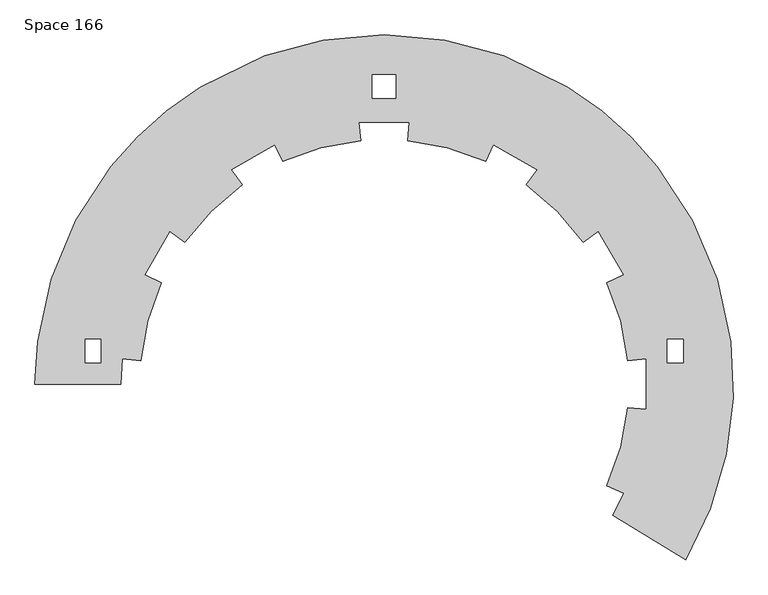
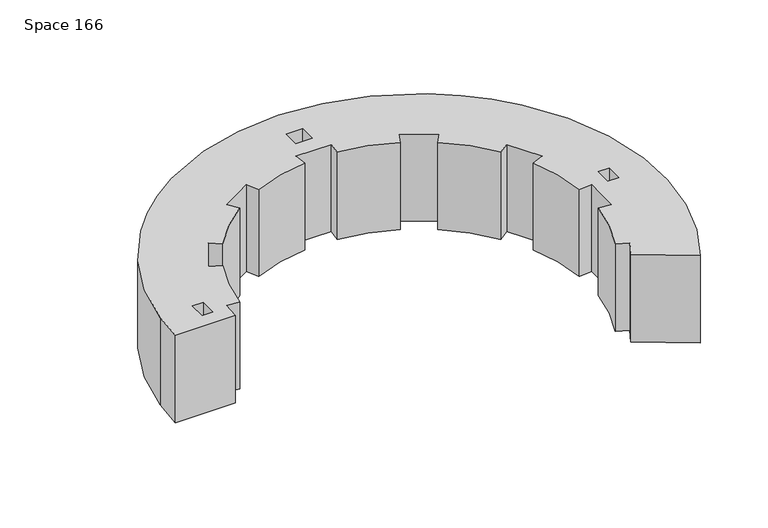
"""IFC4 building model written with IfcOpenShell, lengths in millimetres: proxy geometry, Space 166."""

from ifc_helpers import new_model, si_unit, point, frame_2d, origin, origin_with_axes, place, context, project, spatial, polyline, circle_curve, trimmed, segment, composite_curve, outline, extrude, source, transform, mapped, element, save


def space_166_33292cd7(model_context):
    return source(origin(), model_context, "Body", "SweptSolid", [
        extrude(outline(composite_curve([segment(trimmed(circle_curve(frame_2d((-24639.5440345, -26167.559635)), 5638.8), [point((-19508.4544203, -28505.9318917))], [point((-19026.7039512, -26708.0146643))], True, "CARTESIAN"), True, "CONTINUOUS"), segment(polyline([(-19026.7039512, -26708.0146643), (-18603.2126386, -26748.7922397)]), True, "CONTINUOUS"), segment(trimmed(circle_curve(frame_2d((-24639.5440345, -26167.559635)), 6064.25), [point((-18603.2126386, -26748.7922397))], [point((-18603.2126386, -25586.3270303))], True, "CARTESIAN"), True, "CONTINUOUS"), segment(polyline([(-18603.2126386, -25586.3270303), (-19026.7039512, -25627.1046057)]), True, "CONTINUOUS"), segment(trimmed(circle_curve(frame_2d((-24639.5440345, -26167.559635)), 5638.8), [point((-19026.7039512, -25627.1046057))], [point((-19508.4544203, -23829.1873783))], True, "CARTESIAN"), True, "CONTINUOUS"), segment(polyline([(-19508.4544203, -23829.1873783), (-19121.3113976, -23652.7561382)]), True, "CONTINUOUS"), segment(trimmed(circle_curve(frame_2d((-24639.5440345, -26167.559635)), 6064.25), [point((-19121.3113976, -23652.7561382))], [point((-19702.5440023, -22646.0317359))], True, "CARTESIAN"), True, "CONTINUOUS"), segment(polyline([(-19702.5440023, -22646.0317359), (-20048.9094496, -22893.0918084)]), True, "CONTINUOUS"), segment(trimmed(circle_curve(frame_2d((-24639.5440345, -26167.559635)), 5638.8), [point((-20048.9094496, -22893.0918084))], [point((-21365.0762078, -21576.9250501))], True, "CARTESIAN"), True, "CONTINUOUS"), segment(polyline([(-21365.0762078, -21576.9250501), (-21118.0161353, -21230.5596028)]), True, "CONTINUOUS"), segment(trimmed(circle_curve(frame_2d((-24639.5440345, -26167.559635)), 6064.25), [point((-21118.0161353, -21230.5596028))], [point((-22124.7405377, -20649.3269981))], True, "CARTESIAN"), True, "CONTINUOUS"), segment(polyline([(-22124.7405377, -20649.3269981), (-22301.1717778, -21036.4700208)]), True, "CONTINUOUS"), segment(trimmed(circle_curve(frame_2d((-24639.5440345, -26167.559635)), 5638.8), [point((-22301.1717778, -21036.4700208))], [point((-24099.0890052, -20554.7195517))], True, "CARTESIAN"), True, "CONTINUOUS"), segment(polyline([(-24099.0890052, -20554.7195517), (-24058.3114298, -20131.2282391)]), True, "CONTINUOUS"), segment(trimmed(circle_curve(frame_2d((-24639.5440345, -26167.559635)), 6064.25), [point((-24058.3114298, -20131.2282391))], [point((-25220.7766392, -20131.2282391))], True, "CARTESIAN"), True, "CONTINUOUS"), segment(polyline([(-25220.7766392, -20131.2282391), (-25179.9990638, -20554.7195517)]), True, "CONTINUOUS"), segment(trimmed(circle_curve(frame_2d((-24639.5440345, -26167.559635)), 5638.8), [point((-25179.9990638, -20554.7195517))], [point((-26977.9162912, -21036.4700208))], True, "CARTESIAN"), True, "CONTINUOUS"), segment(polyline([(-26977.9162912, -21036.4700208), (-27154.3475313, -20649.3269981)]), True, "CONTINUOUS"), segment(trimmed(circle_curve(frame_2d((-24639.5440345, -26167.559635)), 6064.25), [point((-27154.3475313, -20649.3269981))], [point((-28161.0719337, -21230.5596028))], True, "CARTESIAN"), True, "CONTINUOUS"), segment(polyline([(-28161.0719337, -21230.5596028), (-27914.0118612, -21576.9250501)]), True, "CONTINUOUS"), segment(trimmed(circle_curve(frame_2d((-24639.5440345, -26167.559635)), 5638.8), [point((-27914.0118612, -21576.9250501))], [point((-29230.1786194, -22893.0918084))], True, "CARTESIAN"), True, "CONTINUOUS"), segment(polyline([(-29230.1786194, -22893.0918084), (-29576.5440667, -22646.0317359)]), True, "CONTINUOUS"), segment(trimmed(circle_curve(frame_2d((-24639.5440345, -26167.559635)), 6064.25), [point((-29576.5440667, -22646.0317359))], [point((-30157.7766714, -23652.7561382))], True, "CARTESIAN"), True, "CONTINUOUS"), segment(polyline([(-30157.7766714, -23652.7561382), (-29770.6336487, -23829.1873783)]), True, "CONTINUOUS"), segment(trimmed(circle_curve(frame_2d((-24639.5440345, -26167.559635)), 5638.8), [point((-29770.6336487, -23829.1873783))], [point((-30252.3841179, -25627.1046057))], True, "CARTESIAN"), True, "CONTINUOUS"), segment(polyline([(-30252.3841179, -25627.1046057), (-30675.8754305, -25586.3270303)]), True, "CONTINUOUS"), segment(trimmed(circle_curve(frame_2d((-24639.5440345, -26167.559635)), 6064.25), [point((-30675.8754305, -25586.3270303))], [point((-30703.7940345, -26167.559635))], True, "CARTESIAN"), True, "CONTINUOUS"), segment(polyline([(-30703.7940345, -26167.559635), (-32684.9940345, -26167.559635)]), True, "CONTINUOUS"), segment(trimmed(circle_curve(frame_2d((-24639.5440345, -26167.559635)), 8045.45), [point((-32684.9940345, -26167.559635))], [point((-32625.0244702, -25187.0659261))], False, "CARTESIAN"), True, "CONTINUOUS"), segment(trimmed(circle_curve(frame_2d((-24639.5440345, -26167.559635)), 8045.45), [point((-32625.0244702, -25187.0659261))], [point((-30935.9788301, -21159.1492517))], False, "CARTESIAN"), True, "CONTINUOUS"), segment(trimmed(circle_curve(frame_2d((-24639.5440345, -26167.559635)), 8045.45), [point((-30935.9788301, -21159.1492517))], [point((-29647.9544178, -19871.1248395))], False, "CARTESIAN"), True, "CONTINUOUS"), segment(trimmed(circle_curve(frame_2d((-24639.5440345, -26167.559635)), 8045.45), [point((-29647.9544178, -19871.1248395))], [point((-28873.1718466, -19326.0933264))], False, "CARTESIAN"), True, "CONTINUOUS"), segment(trimmed(circle_curve(frame_2d((-24639.5440345, -26167.559635)), 8045.45), [point((-28873.1718466, -19326.0933264))], [point((-27391.2499966, -18607.3096391))], False, "CARTESIAN"), True, "CONTINUOUS"), segment(trimmed(circle_curve(frame_2d((-24639.5440345, -26167.559635)), 8045.45), [point((-27391.2499966, -18607.3096391))], [point((-21887.8380724, -18607.3096391))], False, "CARTESIAN"), True, "CONTINUOUS"), segment(trimmed(circle_curve(frame_2d((-24639.5440345, -26167.559635)), 8045.45), [point((-21887.8380724, -18607.3096391))], [point((-20405.9162225, -19326.0933264))], False, "CARTESIAN"), True, "CONTINUOUS"), segment(trimmed(circle_curve(frame_2d((-24639.5440345, -26167.559635)), 8045.45), [point((-20405.9162225, -19326.0933264))], [point((-19631.1336512, -19871.1248395))], False, "CARTESIAN"), True, "CONTINUOUS"), segment(trimmed(circle_curve(frame_2d((-24639.5440345, -26167.559635)), 8045.45), [point((-19631.1336512, -19871.1248395))], [point((-18343.109239, -21159.1492517))], False, "CARTESIAN"), True, "CONTINUOUS"), segment(trimmed(circle_curve(frame_2d((-24639.5440345, -26167.559635)), 8045.45), [point((-18343.109239, -21159.1492517))], [point((-16654.0635988, -25187.0659261))], False, "CARTESIAN"), True, "CONTINUOUS"), segment(trimmed(circle_curve(frame_2d((-24639.5440345, -26167.559635)), 8045.45), [point((-16654.0635988, -25187.0659261))], [point((-17688.4453157, -30218.6696439))], False, "CARTESIAN"), True, "CONTINUOUS"), segment(polyline([(-17688.4453157, -30218.6696439), (-19378.2435507, -29183.1599537)]), True, "CONTINUOUS"), segment(trimmed(circle_curve(frame_2d((-24639.5440345, -26167.559635)), 6064.25), [point((-19378.2435507, -29183.1599537))], [point((-19121.3113976, -28682.3631318))], True, "CARTESIAN"), True, "CONTINUOUS"), segment(polyline([(-19121.3113976, -28682.3631318), (-19508.4544203, -28505.9318917)]), True, "CONTINUOUS")], self_intersect=False), holes=[polyline([(-31164.1690345, -25132.509635), (-31526.1190345, -25132.509635), (-31526.1190345, -25678.609635), (-31164.1690345, -25678.609635), (-31164.1690345, -25132.509635)]), polyline([(-24366.4940345, -19036.509635), (-24912.5940345, -19036.509635), (-24912.5940345, -19582.609635), (-24366.4940345, -19582.609635), (-24366.4940345, -19036.509635)]), polyline([(-17752.9690345, -25132.509635), (-18114.9190345, -25132.509635), (-18114.9190345, -25678.609635), (-17752.9690345, -25678.609635), (-17752.9690345, -25132.509635)])]), origin_with_axes(), (0.0, 0.0, 1.0), 3048.0),
    ])


if __name__ == "__main__":
    model = new_model("IFC4")
    model_context = context("Model", 3, world=origin())
    ifc_project = project(units=[si_unit("LENGTHUNIT", "METRE", prefix="MILLI")], contexts=[model_context])
    site = spatial("IfcSite", under=ifc_project)
    building = spatial("IfcBuilding", under=site)
    placement = place(None, origin())
    space_166_shape = space_166_33292cd7(model_context)
    element("IfcBuildingElementProxy", 1, Name="Space 166", ObjectType="Space 166", at=placement, inside=building, context=model_context, shape_type="MappedRepresentation", body=[
        mapped(space_166_shape, transform((0.0, 0.0, 0.0), x_axis=(1.0, 0.0, 0.0), y_axis=(0.0, 1.0, 0.0), z_axis=(0.0, 0.0, 1.0))),
    ])
    save(model, "model.ifc")

# Revit data of these elements
# Element 1 (IfcBuildingElementProxy, "Space 166")
#   Materials on its faces: "Render Material 255-255-255"
# Materials
#   "Render Material 255-255-255": class "Unassigned", colour RGB 255 255 255, transparency 0
